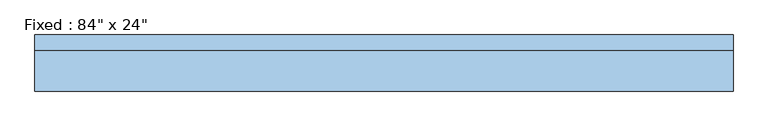
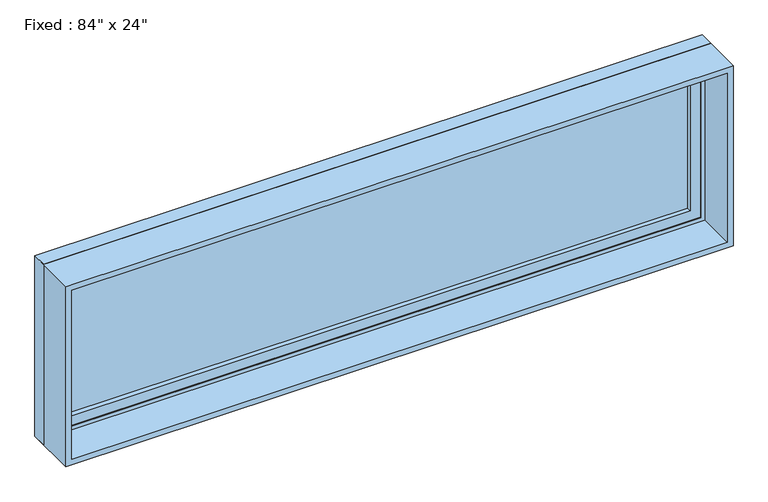
"""IFC4 building model written with IfcOpenShell, lengths in millimetres: window geometry."""

from ifc_helpers import new_model, si_unit, frame, origin, place, context, project, spatial, polyline, outline, extrude, source, transform, mapped, element, save


def window_485a1a53(model_context):
    return source(origin(), model_context, "Body", "SweptSolid", [
        extrude(outline(polyline([(965.2, 93.6625), (965.2, 80.9625), (-1041.4, 80.9625), (-1041.4, 93.6625), (965.2, 93.6625)])), frame((0.0, 0.0, 1282.7), z_axis=(0.0, 0.0, 1.0), x_axis=(1.0, 0.0, 0.0)), (0.0, 0.0, 1.0), 482.6),
        extrude(outline(polyline([(1809.75, -1085.85), (1238.25, -1085.85), (1238.25, 1009.65), (1809.75, 1009.65), (1809.75, -1085.85)]), holes=[polyline([(1765.3, -1041.4), (1765.3, 965.2), (1282.7, 965.2), (1282.7, -1041.4), (1765.3, -1041.4)])]), frame((0.0, 65.0875, 0.0), z_axis=(0.0, 1.0, 0.0), x_axis=(0.0, 0.0, 1.0)), (0.0, 0.0, 1.0), 44.45),
        extrude(outline(polyline([(1828.8, -1104.9), (1219.2, -1104.9), (1219.2, 1028.7), (1828.8, 1028.7), (1828.8, -1104.9)]), holes=[polyline([(1797.05, -1073.15), (1797.05, 996.95), (1250.95, 996.95), (1250.95, -1073.15), (1797.05, -1073.15)])]), frame((0.0, 61.9125, 0.0), z_axis=(0.0, 1.0, 0.0), x_axis=(0.0, 0.0, 1.0)), (0.0, 0.0, 1.0), 47.625),
        extrude(outline(polyline([(1828.8, 1028.7), (1828.8, -1104.9), (1219.2, -1104.9), (1219.2, 1028.7), (1828.8, 1028.7)]), holes=[polyline([(1809.75, 1009.65), (1238.25, 1009.65), (1238.25, -1085.85), (1809.75, -1085.85), (1809.75, 1009.65)])]), frame((0.0, -61.9125, 0.0), z_axis=(0.0, 1.0, 0.0), x_axis=(0.0, 0.0, 1.0)), (0.0, 0.0, 1.0), 171.45),
    ])


if __name__ == "__main__":
    model = new_model("IFC4")
    model_context = context("Model", 3, world=origin())
    ifc_project = project(units=[si_unit("LENGTHUNIT", "METRE", prefix="MILLI")], contexts=[model_context])
    site = spatial("IfcSite", under=ifc_project)
    building = spatial("IfcBuilding", under=site)
    placement = place(None, origin())
    window_shape = window_485a1a53(model_context)
    element("IfcWindow", 1, ObjectType="Fixed : 84\" x 24\"", at=placement, inside=building, context=model_context, shape_type="MappedRepresentation", body=[
        mapped(window_shape, transform((0.0, 0.0, 0.0), x_axis=(1.0, 0.0, 0.0), y_axis=(0.0, 1.0, 0.0), z_axis=(0.0, 0.0, 1.0))),
    ])
    save(model, "model.ifc")

# Revit data of these elements
# Type "Fixed : 84\" x 24\""
#   Type Mark = "20"
#   Construction Type Id = "GSP4R"
#   Assembly Code = "B2020100"
#   Analytic Construction = "1/8 in Pilkington single glazing"
#   Visual Light Transmittance = 0.9
#   Solar Heat Gain Coefficient = 0.78
#   Heat Transfer Coefficient (U) = 3.6886 W/(m²·K)
#   Height = 2' - 0"
#   Default Sill Height = 4' - 0"
#   Width = 7' - 0"
#   Window Inset = 0' - 5"
#   Glass Pane Material = Glass
#   Sash Material = Sash
#   Wall Closure = (empty or 0)
# Element 1 (IfcWindow, "Fixed : 84\" x 24\"")
#   Materials on its faces: "Sash", "Glass"
# Materials
#   "Glass": class "Glass", colour RGB 0 128 192, transparency 0.75, Description = "Soda Lime Glass", Cost = 0
#   "Sash": class "Wood", colour RGB 224 178 126, transparency 0
